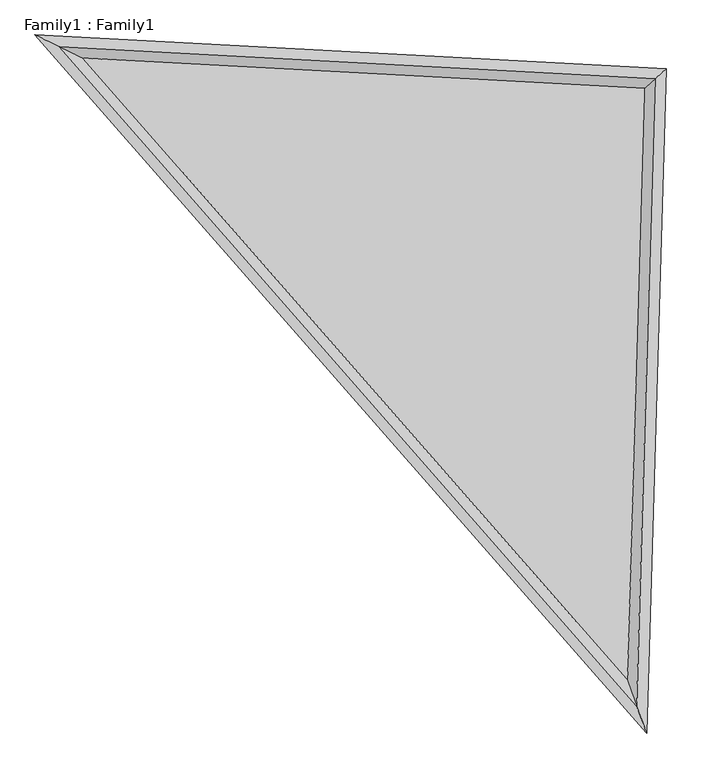
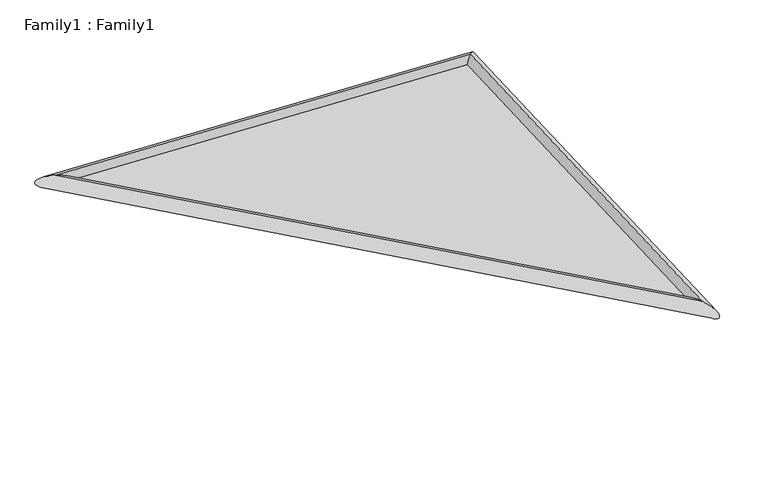
"""IFC4 building model written with IfcOpenShell, lengths in millimetres: proxy geometry, Family1 : Family1."""

from ifc_helpers import new_model, si_unit, frame, origin, origin_with_axes, place, context, project, spatial, polyline, ellipse_curve, outline, extrude, source, transform, mapped, element, save
from ifc_brep_helpers import cylinder_surface, advanced_brep


def family1_family1_7222e5bf(model_context):
    return source(origin(), model_context, "Body", "SolidModel", [
        extrude(outline(polyline([(2688.2734843, -3601.1650368), (-2783.3817957, 2644.3016013), (2862.0307624, 2340.8046403), (2688.2734843, -3601.1650368)])), origin_with_axes(), (0.0, 0.0, 1.0), 34.1328789),
        advanced_brep(
        [(2688.2734843, -3601.1650368, 100.0), (2688.2734843, -3601.1650368, -100.0), (-2783.3817957, 2644.3016013, -100.0), (-2783.3817957, 2644.3016013, 100.0), (2862.0307624, 2340.8046403, -100.0), (2862.0307624, 2340.8046403, 100.0)],
        [
            (0, 1, ellipse_curve(frame((2688.2734843, -3601.1650368, 0.0), z_axis=(-0.9410384470925119, -0.3382996321217535, 0.0), x_axis=(0.33829963212175346, -0.9410384470925119, 0.0)), 273.4769585, 100.0)),
            (1, 2),
            (2, 3, ellipse_curve(frame((-2783.3817957, 2644.3016013, 0.0), z_axis=(-0.4372385407160553, -0.8993455723538614, 0.0), x_axis=(0.8993455723538614, -0.4372385407160552, 0.0)), 257.5135809, 100.0)),
            (3, 0),
            (1, 0, ellipse_curve(frame((2688.2734843, -3601.1650368, 0.0), z_axis=(-0.9410384470925119, -0.3382996321217535, 0.0), x_axis=(0.33829963212175346, -0.9410384470925119, 0.0)), 273.4769585, 100.0)),
            (3, 2, ellipse_curve(frame((-2783.3817957, 2644.3016013, 0.0), z_axis=(-0.4372385407160553, -0.8993455723538614, 0.0), x_axis=(0.8993455723538614, -0.4372385407160552, 0.0)), 257.5135809, 100.0)),
            (2, 4),
            (4, 5, ellipse_curve(frame((2862.0307624, 2340.8046403, 0.0), z_axis=(-0.677182694115907, 0.7358149215597097, 0.0), x_axis=(-0.7358149215597097, -0.677182694115907, 0.0)), 139.7220683, 100.0)),
            (5, 3),
            (5, 4, ellipse_curve(frame((2862.0307624, 2340.8046403, 0.0), z_axis=(-0.677182694115907, 0.7358149215597097, 0.0), x_axis=(-0.7358149215597097, -0.677182694115907, 0.0)), 139.7220683, 100.0)),
            (4, 1),
            (0, 5),
        ],
        [
            cylinder_surface(frame((2688.2734843, -3601.1650368, 0.0), z_axis=(0.6589732200408903, -0.7521664013161852, 0.0), x_axis=(-0.7521664013161852, -0.6589732200408903, 0.0)), 100.0),
            cylinder_surface(frame((-2783.3817957, 2644.3016013, 0.0), z_axis=(-0.9985580599747563, 0.05368240735521368, 0.0), x_axis=(0.05368240735521368, 0.9985580599747563, 0.0)), 100.0),
            cylinder_surface(frame((2862.0307624, 2340.8046403, 0.0), z_axis=(0.02922987559125797, 0.999572715900609, 0.0), x_axis=(0.999572715900609, -0.02922987559125797, 0.0)), 100.0),
        ],
        [
            (0, [[1, 2, 3, 4]]),
            (0, [[5, -4, 6, -2]]),
            (1, [[-3, 7, 8, 9]]),
            (1, [[-6, -9, 10, -7]]),
            (2, [[-8, 11, -1, 12]]),
            (2, [[-10, -12, -5, -11]]),
        ],
    ),
    ])


if __name__ == "__main__":
    model = new_model("IFC4")
    model_context = context("Model", 3, world=origin())
    ifc_project = project(units=[si_unit("LENGTHUNIT", "METRE", prefix="MILLI")], contexts=[model_context])
    site = spatial("IfcSite", under=ifc_project)
    building = spatial("IfcBuilding", under=site)
    placement = place(None, origin())
    family1_family1_shape = family1_family1_7222e5bf(model_context)
    element("IfcBuildingElementProxy", 1, Name="Family1 : Family1", ObjectType="Family1 : Family1", at=placement, inside=building, context=model_context, shape_type="MappedRepresentation", body=[
        mapped(family1_family1_shape, transform((0.0, 0.0, 0.0), x_axis=(1.0, 0.0, 0.0), y_axis=(0.0, 1.0, 0.0), z_axis=(0.0, 0.0, 1.0))),
    ])
    save(model, "model.ifc")

# Revit data of these elements
# Type "Family1 : Family1"
#   Default Elevation = 0
# Element 1 (IfcBuildingElementProxy, "Family1 : Family1")
#   Materials on its faces: "Glass"
# Materials
#   "Glass": class "Glass", colour RGB 0 128 192, transparency 0.9, Description = "Soda Lime Glass", Cost = 0
